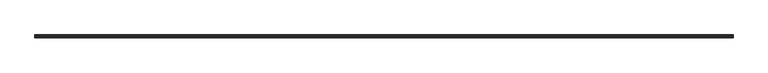
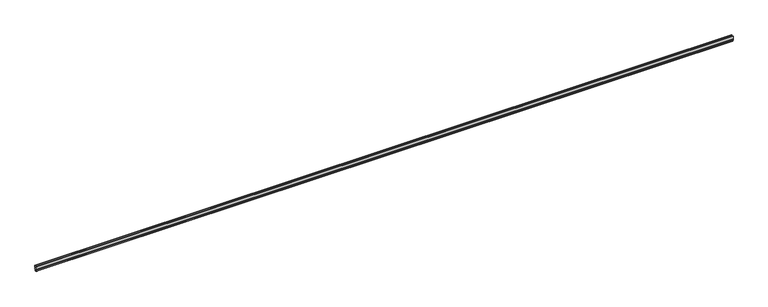
"""IFC4 building model written with IfcOpenShell, lengths in millimetres: proxy geometry, Generic Models 6:Generic Models 2:318829:Generic Models 2:318829 : Generic Models 6:Generic Models 2:318829:23 : Generic Models 6:Generic Models 2:318829:Generic Models 2:318829 : Generic Models 6:Generic Models 2:318829:300683."""

from ifc_helpers import new_model, si_unit, frame, origin, place, context, project, spatial, polyline, outline, extrude, source, transform, mapped, element, save


def generic_models_f3fa0046(model_context):
    return source(origin(), model_context, "Body", "SweptSolid", [
        extrude(outline(polyline([(-568195.519054, 4989.8384868), (-568195.519054, 4998.640625), (-568194.0704092, 4998.0745121), (-568190.756554, 4997.603983), (-568187.4426988, 4998.0745121), (-568185.994054, 4998.640625), (-568185.994054, 4989.8384868), (-568187.3182372, 4992.2283119), (-568189.1803134, 4993.6896194), (-568191.2889778, 4993.9938013), (-568193.3143495, 4993.093271), (-568194.9395776, 4991.1289083), (-568195.519054, 4989.8384868)])), frame((591391.6367242, 0.0, 0.0), z_axis=(1.0, 0.0, 0.0), x_axis=(0.0, 1.0, 0.0)), (0.0, 0.0, 1.0), 2438.4),
        extrude(outline(polyline([(-568195.3996482, 4984.7034115), (-568195.519054, 4986.2930455), (-568195.3996482, 4987.8826794), (-568194.4800264, 4990.7471007), (-568192.8229253, 4992.7293418), (-568190.756554, 4993.4367955), (-568188.6901827, 4992.7293418), (-568187.0330816, 4990.7471007), (-568186.1134598, 4987.8826794), (-568185.994054, 4986.2930455), (-568186.1134598, 4984.7034115), (-568187.0330816, 4981.8389902), (-568188.6901827, 4979.8567491), (-568190.756554, 4979.1492955), (-568192.8229253, 4979.8567491), (-568194.4800264, 4981.8389902), (-568195.3996482, 4984.7034115)])), frame((591391.6367242, 0.0, 0.0), z_axis=(1.0, 0.0, 0.0), x_axis=(0.0, 1.0, 0.0)), (0.0, 0.0, 1.0), 2438.4),
    ])


if __name__ == "__main__":
    model = new_model("IFC4")
    model_context = context("Model", 3, world=origin())
    ifc_project = project(units=[si_unit("LENGTHUNIT", "METRE", prefix="MILLI")], contexts=[model_context])
    site = spatial("IfcSite", under=ifc_project)
    building = spatial("IfcBuilding", under=site)
    placement = place(None, origin())
    generic_models_shape = generic_models_f3fa0046(model_context)
    element("IfcBuildingElementProxy", 1, Name="Generic Models 6:Generic Models 2:318829:Generic Models 2:318829 : Generic Models 6:Generic Models 2:318829:23 : Generic Models 6:Generic Models 2:318829:Generic Models 2:318829 : Generic Models 6:Generic Models 2:318829:300683", ObjectType="Generic Models 6:Generic Models 2:318829:Generic Models 2:318829 : Generic Models 6:Generic Models 2:318829:23 : Generic Models 6:Generic Models 2:318829:Generic Models 2:318829 : Generic Models 6:Generic Models 2:318829:300683", at=placement, inside=building, context=model_context, shape_type="MappedRepresentation", body=[
        mapped(generic_models_shape, transform((0.0, 0.0, 0.0), x_axis=(1.0, 0.0, 0.0), y_axis=(0.0, 1.0, 0.0), z_axis=(0.0, 0.0, 1.0))),
    ])
    save(model, "model.ifc")

# Revit data of these elements
# Type "Generic Models 6:Generic Models 2:318829:Generic Models 2:318829 : Generic Models 6:Generic Models 2:318829:23 : Generic Models 6:Generic Models 2:318829:Generic Models 2:318829 : Generic Models 6:Generic Models 2:318829:300683"
#   NameOverride = "Generic Models 6:Generic Models 2:318829:Generic Models 2:318829 : Generic Models 6:Generic Models 2:318829:300683"
#   ObjectTypeOverride = "Generic Models 2:318829 : Generic Models 6:Generic Models 2:318829"
#   Reference = "Generic Models 2"
#   Tag = "300683"
# Element 1 (IfcBuildingElementProxy, "Generic Models 6:Generic Models 2:318829:Generic Models 2:318829 : Generic Models 6:Generic Models 2:318829:23 : Generic Models 6:Generic Models 2:318829:Generic Models 2:318829 : Generic Models 6:Generic Models 2:318829:300683")
#   Materials on its faces: "SEALANT & BACKER ROD, IF NECESSARY"
# Materials
#   "SEALANT & BACKER ROD, IF NECESSARY": class "Unassigned", colour RGB 120 120 120, transparency 0, Cost = 0
